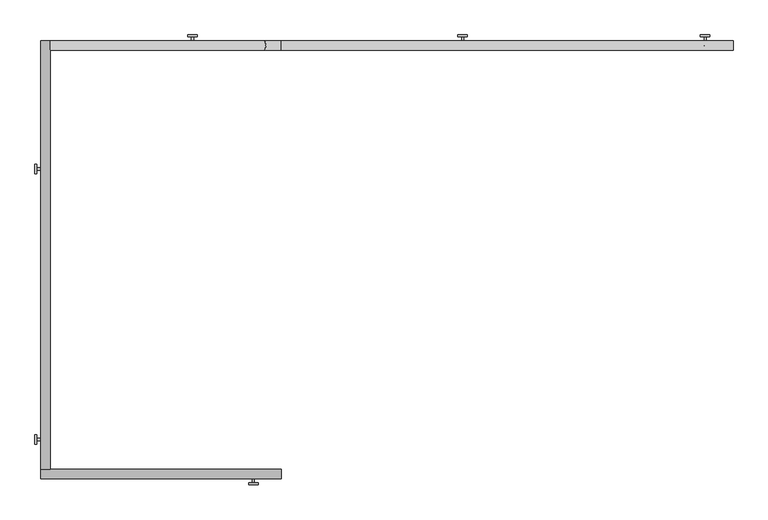
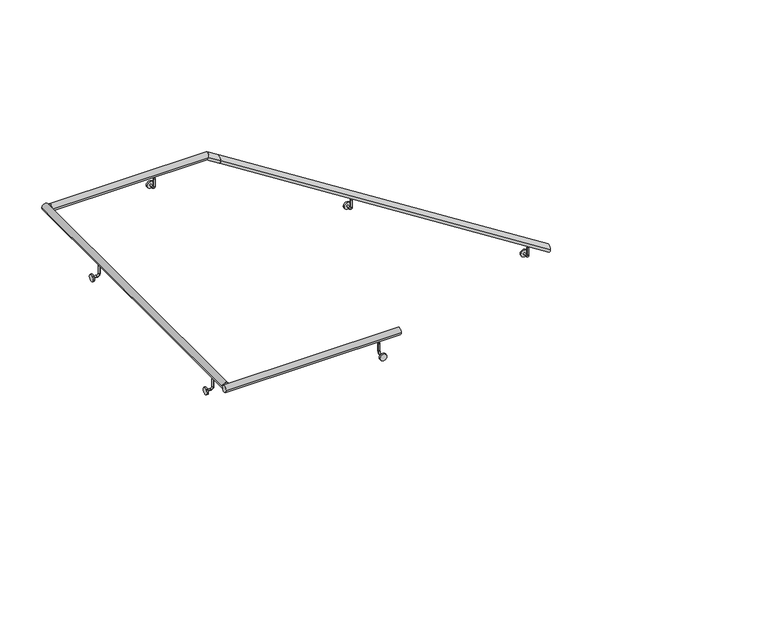
"""IFC4 building model written with IfcOpenShell, lengths in millimetres: railing geometry."""

import ifcopenshell
import ifcopenshell.guid

model = None  # the IFC model being written
_history = None  # IfcOwnerHistory: only IFC2X3 demands one
_inside = {}  # id of a spatial element -> (the spatial element, [elements in it])
_under = {}  # id of a project, library or spatial element -> (it, [spatial elements below it])
_declared = {}  # id of a project -> (the project, [libraries it declares])
_typed = {}  # id of a type object -> (the type object, [elements of that type])
_made_of = {}  # id of a material, layer set ... -> (it, [elements and type objects made of it])


def new_model(schema):
    """Start an empty IFC model of exactly this schema.

    Asked for "IFC4X3", IfcOpenShell would pick the latest addendum, in which some entities
    have other attributes; the version numbers below select the first issue.
    IFC2X3 requires an IfcOwnerHistory on every rooted entity: one is made here for all.
    """
    global model, _history
    if schema == "IFC4X3":
        model = ifcopenshell.file(schema_version=(4, 3, 0, 0))
    else:
        model = ifcopenshell.file(schema=schema)
    _inside.clear()
    _under.clear()
    _declared.clear()
    _typed.clear()
    _made_of.clear()
    _history = None
    if model.schema == "IFC2X3":
        org = make("IfcOrganization", Name="unknown")
        user = make(
            "IfcPersonAndOrganization",
            ThePerson=make("IfcPerson", FamilyName="unknown"),
            TheOrganization=org,
        )
        app = make(
            "IfcApplication",
            ApplicationDeveloper=org,
            Version="unknown",
            ApplicationFullName="unknown",
            ApplicationIdentifier="unknown",
        )
        _history = make(
            "IfcOwnerHistory",
            OwningUser=user,
            OwningApplication=app,
            ChangeAction="ADDED",
            CreationDate=0,
        )
    return model


def make(cls, **values):
    """One entity of the class cls with the attributes given. An attribute that is None is left unset."""
    return model.create_entity(
        cls, **{name: value for name, value in values.items() if value is not None}
    )


def rooted(cls, **values):
    """An entity with a GlobalId (a new one), such as an element, a storey or a relation."""
    return make(cls, GlobalId=ifcopenshell.guid.new(), OwnerHistory=_history, **values)


def si_unit(unit_type, name, prefix=None):
    """IfcSIUnit, for example si_unit("LENGTHUNIT", "METRE", prefix="MILLI")."""
    return make("IfcSIUnit", UnitType=unit_type, Prefix=prefix, Name=name)


def assignment(units):
    """IfcUnitAssignment: the units of a project."""
    return None if units is None else make("IfcUnitAssignment", Units=units)


def point(xyz):
    """IfcCartesianPoint."""
    return None if xyz is None else make("IfcCartesianPoint", Coordinates=xyz)


def direction(xyz):
    """IfcDirection."""
    return None if xyz is None else make("IfcDirection", DirectionRatios=xyz)


def frame(location, z_axis=None, x_axis=None):
    """IfcAxis2Placement3D, a coordinate frame: its origin and axes. An axis left out is left unset."""
    return make(
        "IfcAxis2Placement3D",
        Location=point(location),
        Axis=direction(z_axis),
        RefDirection=direction(x_axis),
    )


def frame_2d(location, x_axis=None):
    """IfcAxis2Placement2D, a coordinate frame in the plane: its origin and x axis."""
    return make(
        "IfcAxis2Placement2D", Location=point(location), RefDirection=direction(x_axis)
    )


def origin():
    """The frame at (0, 0, 0) with its axes left unset."""
    return frame((0.0, 0.0, 0.0))


def place(relative_to, where):
    """IfcLocalPlacement: puts the frame where relative to a parent placement (None: the world)."""
    return make(
        "IfcLocalPlacement", PlacementRelTo=relative_to, RelativePlacement=where
    )


def context(
    kind, dimensions, precision=None, world=None, true_north=None, identifier=None
):
    """IfcGeometricRepresentationContext, for example the 3D "Model" context."""
    return make(
        "IfcGeometricRepresentationContext",
        ContextIdentifier=identifier,
        ContextType=kind,
        CoordinateSpaceDimension=dimensions,
        Precision=precision,
        WorldCoordinateSystem=world,
        TrueNorth=true_north,
    )


def project(units=None, contexts=None):
    """IfcProject with its units and contexts."""
    return rooted(
        "IfcProject",
        Name="project",
        RepresentationContexts=contexts,
        UnitsInContext=assignment(units),
    )


def spatial(cls, under=None, at=None, **own):
    """A site, building, storey or space (cls), placed at a placement, below another one or the project."""
    s = rooted(cls, ObjectPlacement=at, **own)
    if under is not None:
        _under.setdefault(under.id(), (under, []))[1].append(s)
    return s


def circle_curve(where, radius):
    """IfcCircle in the frame where."""
    return make("IfcCircle", Position=where, Radius=radius)


def ellipse_curve(where, semi_axis1, semi_axis2):
    """IfcEllipse in the frame where."""
    return make(
        "IfcEllipse", Position=where, SemiAxis1=semi_axis1, SemiAxis2=semi_axis2
    )


def trimmed(basis, trim1, trim2, sense, master):
    """IfcTrimmedCurve: the piece of a basis curve between two trims."""
    return make(
        "IfcTrimmedCurve",
        BasisCurve=basis,
        Trim1=trim1,
        Trim2=trim2,
        SenseAgreement=sense,
        MasterRepresentation=master,
    )


def segment(curve, same_sense, transition):
    """IfcCompositeCurveSegment."""
    return make(
        "IfcCompositeCurveSegment",
        Transition=transition,
        SameSense=same_sense,
        ParentCurve=curve,
    )


def composite_curve(segments, self_intersect=None):
    """IfcCompositeCurve: segments joined end to end."""
    return make("IfcCompositeCurve", Segments=segments, SelfIntersect=self_intersect)


def outline(outer, holes=None, kind="AREA"):
    """IfcArbitraryClosedProfileDef: a profile drawn as a closed curve; with holes, ...WithVoids."""
    if holes is None:
        return make("IfcArbitraryClosedProfileDef", ProfileType=kind, OuterCurve=outer)
    return make(
        "IfcArbitraryProfileDefWithVoids",
        ProfileType=kind,
        OuterCurve=outer,
        InnerCurves=holes,
    )


def extrude(swept, where, along, depth):
    """IfcExtrudedAreaSolid: the profile swept, set in the frame where, extruded along a direction by depth."""
    return make(
        "IfcExtrudedAreaSolid",
        SweptArea=swept,
        Position=where,
        ExtrudedDirection=direction(along),
        Depth=depth,
    )


def shape(context_of_items, identifier, shape_type, items):
    """IfcShapeRepresentation: the items that make up one representation, for example the "Body"."""
    return make(
        "IfcShapeRepresentation",
        ContextOfItems=context_of_items,
        RepresentationIdentifier=identifier,
        RepresentationType=shape_type,
        Items=items,
    )


def source(mapping_origin, context_of_items, identifier, shape_type, items):
    """IfcRepresentationMap: a shape defined once, which mapped items show again and again."""
    return make(
        "IfcRepresentationMap",
        MappingOrigin=mapping_origin,
        MappedRepresentation=shape(context_of_items, identifier, shape_type, items),
    )


def transform(
    local_origin,
    x_axis=None,
    y_axis=None,
    z_axis=None,
    scale=None,
    scale2=None,
    scale3=None,
    uniform=True,
):
    """IfcCartesianTransformationOperator3D, or its non-uniform kind. x_axis, y_axis, z_axis: its Axis1, 2, 3."""
    if uniform:
        return make(
            "IfcCartesianTransformationOperator3D",
            Axis1=direction(x_axis),
            Axis2=direction(y_axis),
            LocalOrigin=point(local_origin),
            Scale=scale,
            Axis3=direction(z_axis),
        )
    return make(
        "IfcCartesianTransformationOperator3DnonUniform",
        Axis1=direction(x_axis),
        Axis2=direction(y_axis),
        LocalOrigin=point(local_origin),
        Scale=scale,
        Axis3=direction(z_axis),
        Scale2=scale2,
        Scale3=scale3,
    )


def mapped(mapping_source, mapping_target):
    """IfcMappedItem: shows the shape of a source again, moved by a transform."""
    return make(
        "IfcMappedItem", MappingSource=mapping_source, MappingTarget=mapping_target
    )


def made_of(thing, what):
    """Note that an element or type object is made of a material, layer set ...; save() writes the relation."""
    if what is not None:
        _made_of.setdefault(what.id(), (what, []))[1].append(thing)
    return thing


def element(
    cls,
    number,
    at=None,
    inside=None,
    cuts=None,
    type_object=None,
    material=None,
    context=None,
    identifier="Body",
    shape_type=None,
    held_by="IfcProductDefinitionShape",
    body=None,
    shapes=None,
    **own,
):
    """One element of the class cls, such as IfcWall. Its Tag is "e" and its number.

    at: its placement. inside: the storey or other place that contains it. cuts: it is an
    opening in that element (IfcRelVoidsElement). A single representation is given by context,
    identifier, shape_type and body (its items); several are given by shapes. held_by: the class
    of the entity that holds the representations. save() writes the other relations.
    """
    e = rooted(cls, Tag="e%d" % number, ObjectPlacement=at, **own)
    if body is not None:
        shapes = [shape(context, identifier, shape_type, body)]
    if shapes is not None:
        e.Representation = make(held_by, Representations=shapes)
    if inside is not None:
        _inside.setdefault(inside.id(), (inside, []))[1].append(e)
    if cuts is not None:
        rooted(
            "IfcRelVoidsElement", RelatingBuildingElement=cuts, RelatedOpeningElement=e
        )
    if type_object is not None:
        _typed.setdefault(type_object.id(), (type_object, []))[1].append(e)
    return made_of(e, material)


def aggregate(whole, parts):
    """IfcRelAggregates: a whole, such as a stair, and the parts it consists of."""
    return rooted("IfcRelAggregates", RelatingObject=whole, RelatedObjects=parts)


def save(model, path):
    """Write the relations noted so far, then the file.

    IfcRelAggregates (storeys below a building ...), IfcRelContainedInSpatialStructure (elements
    in a storey), IfcRelDefinesByType, IfcRelAssociatesMaterial and IfcRelDeclares: one each for
    every whole, place, type object, material and project.
    """
    for whole, parts in _under.values():
        aggregate(whole, parts)
    for where, things in _inside.values():
        rooted(
            "IfcRelContainedInSpatialStructure",
            RelatedElements=things,
            RelatingStructure=where,
        )
    for kind, things in _typed.values():
        rooted("IfcRelDefinesByType", RelatedObjects=things, RelatingType=kind)
    for what, things in _made_of.values():
        rooted("IfcRelAssociatesMaterial", RelatedObjects=things, RelatingMaterial=what)
    for by, libraries in _declared.values():
        rooted("IfcRelDeclares", RelatingContext=by, RelatedDefinitions=libraries)
    model.write(path)


def plane_surface(at):
    """IfcPlane: the flat surface through the origin of the frame at, square to its z axis."""
    return make("IfcPlane", Position=at)


def cylinder_surface(at, radius):
    """IfcCylindricalSurface: all points at the distance radius from the z axis of the frame at."""
    return make("IfcCylindricalSurface", Position=at, Radius=radius)


def revolved_surface(curve, axis_point, axis_direction):
    """IfcSurfaceOfRevolution: the curve turned about the line through axis_point along axis_direction."""
    return make(
        "IfcSurfaceOfRevolution",
        SweptCurve=make("IfcArbitraryOpenProfileDef", ProfileType="CURVE", Curve=curve),
        AxisPosition=make("IfcAxis1Placement", Location=point(axis_point), Axis=direction(axis_direction)),
    )


def advanced_brep(points, edges, surfaces, faces):
    """IfcAdvancedBrep: a solid bounded by faces that lie on surfaces and meet in shared edges.

    An edge is (start, end): straight between two places in points (the first is 0);
    or (start, end, curve); or (start, end, curve, False) where it runs against its curve.
    A face is (place in surfaces, loops), or (place, loops, False) where it looks against
    its surface's normal. A loop lists edges by number (the first is 1), with a minus sign
    where the edge is run from its end to its start. The first loop is the outer one.
    """
    corners = [point(p) for p in points]
    vertices = [make("IfcVertexPoint", VertexGeometry=c) for c in corners]
    made = []
    for start, end, *more in edges:
        made.append(
            make(
                "IfcEdgeCurve",
                EdgeStart=vertices[start],
                EdgeEnd=vertices[end],
                EdgeGeometry=more[0] if more else make("IfcPolyline", Points=[corners[start], corners[end]]),
                SameSense=more[1] if len(more) > 1 else True,
            )
        )
    hull = []
    for where, loops, *sense in faces:
        bounds = []
        for j, loop in enumerate(loops):
            ring = [make("IfcOrientedEdge", EdgeElement=made[abs(k) - 1], Orientation=k > 0) for k in loop]
            bounds.append(
                make(
                    "IfcFaceOuterBound" if j == 0 else "IfcFaceBound",
                    Bound=make("IfcEdgeLoop", EdgeList=ring),
                    Orientation=True,
                )
            )
        hull.append(make("IfcAdvancedFace", Bounds=bounds, FaceSurface=surfaces[where], SameSense=sense[0] if sense else True))
    return make("IfcAdvancedBrep", Outer=make("IfcClosedShell", CfsFaces=hull))


def railing_d584f0b8(model_context):
    return source(origin(), model_context, "Body", "SolidModel", [
        advanced_brep(
        [(-47747.4858495, 17739.1574868, 4652.1467196), (-47747.4858495, 17789.1574868, 4652.1467196), (-50177.4858495, 17739.1574868, 6195.0038624), (-50177.4858495, 17789.1574868, 6195.0038624)],
        [
            (0, 1, ellipse_curve(frame((-47747.4858495, 17764.1574868, 4652.1467196), z_axis=(1.0, 0.0, 0.0), x_axis=(0.0, 0.0, -1.0)), 29.613386, 25.0)),
            (1, 0, ellipse_curve(frame((-47747.4858495, 17764.1574868, 4652.1467196), z_axis=(1.0, 0.0, 0.0), x_axis=(0.0, 0.0, -1.0)), 29.613386, 25.0)),
            (2, 3, ellipse_curve(frame((-50177.4858495, 17764.1574868, 6195.0038624), z_axis=(-1.0, 0.0, 0.0), x_axis=(0.0, 0.0, -1.0)), 29.613386, 25.0)),
            (3, 2, ellipse_curve(frame((-50177.4858495, 17764.1574868, 6195.0038624), z_axis=(-1.0, 0.0, 0.0), x_axis=(0.0, 0.0, -1.0)), 29.613386, 25.0)),
            (0, 2),
            (3, 1),
        ],
        [
            plane_surface(frame((-47747.4858495, 17764.1574868, 4681.7601056), z_axis=(1.0, 0.0, 0.0), x_axis=(0.0, -1.0, 0.0))),
            plane_surface(frame((-50177.4858495, 17764.1574868, 6224.6172485), z_axis=(-1.0, 0.0, 0.0), x_axis=(0.0, -1.0, 0.0))),
            cylinder_surface(frame((-47760.8860529, 17764.1574868, 4660.6547852), z_axis=(0.8442128152478047, 0.0, -0.5360081366652713), x_axis=(0.0, 1.0, 0.0)), 25.0),
        ],
        [
            (0, [[1, 2]]),
            (1, [[3, 4]]),
            (2, [[-1, 5, -4, 6]]),
            (2, [[-2, -6, -3, -5]]),
        ],
    ),
        advanced_brep(
        [(-50177.4858495, 17739.1574868, 6195.0038624), (-50177.4858495, 17789.1574868, 6195.0038624), (-50268.4797662, 17739.1574868, 6252.7777778), (-50268.4797662, 17789.1574868, 6252.7777778), (-51419.7848926, 17739.1574868, 6252.7777778), (-51419.7848926, 17789.1574868, 6252.7777778)],
        [
            (0, 1, ellipse_curve(frame((-50177.4858495, 17764.1574868, 6195.0038624), z_axis=(1.0, 0.0, 0.0), x_axis=(0.0, 0.0, -1.0)), 29.613386, 25.0)),
            (1, 0, ellipse_curve(frame((-50177.4858495, 17764.1574868, 6195.0038624), z_axis=(1.0, 0.0, 0.0), x_axis=(0.0, 0.0, -1.0)), 29.613386, 25.0)),
            (0, 2),
            (2, 3, ellipse_curve(frame((-50268.4797662, 17764.1574868, 6252.7777778), z_axis=(0.9602637177483601, 0.0, -0.27909423565544655), x_axis=(-0.2790942356554468, 0.0, -0.9602637177483601)), 26.0345148, 25.0)),
            (3, 1),
            (3, 2, ellipse_curve(frame((-50268.4797662, 17764.1574868, 6252.7777778), z_axis=(0.9602637177483601, 0.0, -0.27909423565544655), x_axis=(-0.2790942356554468, 0.0, -0.9602637177483601)), 26.0345148, 25.0)),
            (4, 5, circle_curve(frame((-51419.7848926, 17764.1574868, 6252.7777778), z_axis=(-1.0, 0.0, 0.0), x_axis=(0.0, 1.0, 0.0)), 25.0)),
            (5, 4, circle_curve(frame((-51419.7848926, 17764.1574868, 6252.7777778), z_axis=(-1.0, 0.0, 0.0), x_axis=(0.0, 1.0, 0.0)), 25.0)),
            (2, 4),
            (5, 3),
        ],
        [
            plane_surface(frame((-50177.4858495, 17764.1574868, 6224.6172485), z_axis=(1.0, 0.0, 0.0), x_axis=(0.0, -1.0, 0.0))),
            cylinder_surface(frame((-50190.8860529, 17764.1574868, 6203.5119281), z_axis=(0.844212815247804, 0.0, -0.5360081366652723), x_axis=(0.0, 1.0, 0.0)), 25.0),
            plane_surface(frame((-51419.7848926, 17764.1574868, 6277.7777778), z_axis=(-1.0, 0.0, 0.0), x_axis=(0.0, -1.0, 0.0))),
            cylinder_surface(frame((-50261.2136831, 17764.1574868, 6252.7777778), z_axis=(1.0, 0.0, 0.0), x_axis=(0.0, 1.0, 0.0)), 25.0),
        ],
        [
            (0, [[1, 2]]),
            (1, [[-1, 3, 4, 5]]),
            (1, [[-2, -5, 6, -3]]),
            (2, [[7, 8]]),
            (3, [[-4, 9, -8, 10]]),
            (3, [[-6, -10, -7, -9]]),
        ],
    ),
        advanced_brep(
        [(-51419.7848926, 17789.1574868, 6252.7777778), (-51469.7848926, 17789.1574868, 6252.7777778), (-51419.7848926, 15484.3574868, 6252.7777778), (-51469.7848926, 15484.3574868, 6252.7777778)],
        [
            (0, 1, circle_curve(frame((-51444.7848926, 17789.1574868, 6252.7777778), z_axis=(0.0, 1.0, 0.0), x_axis=(-1.0, 0.0, 0.0)), 25.0)),
            (1, 0, circle_curve(frame((-51444.7848926, 17789.1574868, 6252.7777778), z_axis=(0.0, 1.0, 0.0), x_axis=(-1.0, 0.0, 0.0)), 25.0)),
            (2, 3, circle_curve(frame((-51444.7848926, 15484.3574868, 6252.7777778), z_axis=(0.0, -1.0, 0.0), x_axis=(-1.0, 0.0, 0.0)), 25.0)),
            (3, 2, circle_curve(frame((-51444.7848926, 15484.3574868, 6252.7777778), z_axis=(0.0, -1.0, 0.0), x_axis=(-1.0, 0.0, 0.0)), 25.0)),
            (0, 2),
            (3, 1),
        ],
        [
            plane_surface(frame((-51444.7848926, 17789.1574868, 6277.7777778), z_axis=(0.0, 1.0, 0.0), x_axis=(0.0, 0.0, -1.0))),
            plane_surface(frame((-51444.7848926, 15484.3574868, 6277.7777778), z_axis=(0.0, -1.0, 0.0), x_axis=(0.0, 0.0, -1.0))),
            cylinder_surface(frame((-51444.7848926, 17789.1574868, 6252.7777778), z_axis=(0.0, 1.0, 0.0), x_axis=(-1.0, 0.0, 0.0)), 25.0),
        ],
        [
            (0, [[1, 2]]),
            (1, [[3, 4]]),
            (2, [[-1, 5, -4, 6]]),
            (2, [[-2, -6, -3, -5]]),
        ],
    ),
        advanced_brep(
        [(-51469.7848926, 15484.3574868, 6252.7777778), (-51469.7848926, 15434.3574868, 6252.7777778), (-50177.4858495, 15484.3574868, 6252.7777778), (-50177.4858495, 15434.3574868, 6252.7777778)],
        [
            (0, 1, circle_curve(frame((-51469.7848926, 15459.3574868, 6252.7777778), z_axis=(-1.0, 0.0, 0.0), x_axis=(0.0, -1.0, 0.0)), 25.0)),
            (1, 0, circle_curve(frame((-51469.7848926, 15459.3574868, 6252.7777778), z_axis=(-1.0, 0.0, 0.0), x_axis=(0.0, -1.0, 0.0)), 25.0)),
            (2, 3, circle_curve(frame((-50177.4858495, 15459.3574868, 6252.7777778), z_axis=(1.0, 0.0, 0.0), x_axis=(0.0, -1.0, 0.0)), 25.0)),
            (3, 2, circle_curve(frame((-50177.4858495, 15459.3574868, 6252.7777778), z_axis=(1.0, 0.0, 0.0), x_axis=(0.0, -1.0, 0.0)), 25.0)),
            (0, 2),
            (3, 1),
        ],
        [
            plane_surface(frame((-51469.7848926, 15459.3574868, 6277.7777778), z_axis=(-1.0, 0.0, 0.0), x_axis=(0.0, 1.0, 0.0))),
            plane_surface(frame((-50177.4858495, 15459.3574868, 6277.7777778), z_axis=(1.0, 0.0, 0.0), x_axis=(0.0, 1.0, 0.0))),
            cylinder_surface(frame((-51469.7848926, 15459.3574868, 6252.7777778), z_axis=(-1.0, 0.0, 0.0), x_axis=(0.0, -1.0, 0.0)), 25.0),
        ],
        [
            (0, [[1, 2]]),
            (1, [[3, 4]]),
            (2, [[-1, 5, -4, 6]]),
            (2, [[-2, -6, -3, -5]]),
        ],
    ),
        advanced_brep(
        [(-51444.7848926, 15652.288061, 6208.7277778), (-51444.7848926, 15639.588061, 6208.7277778), (-51444.7848926, 15652.288061, 6151.5777778), (-51444.7848926, 15639.588061, 6151.5777778), (-51463.8348926, 15639.588061, 6132.5277778), (-51463.8348926, 15652.288061, 6132.5277778), (-51492.4098926, 15652.288061, 6132.5277778), (-51492.4098926, 15639.588061, 6132.5277778)],
        [
            (0, 1, circle_curve(frame((-51444.7848926, 15645.938061, 6208.7277778), z_axis=(0.0, 0.0, 1.0), x_axis=(0.0, -1.0, 0.0)), 6.35)),
            (1, 0, circle_curve(frame((-51444.7848926, 15645.938061, 6208.7277778), z_axis=(0.0, 0.0, 1.0), x_axis=(0.0, -1.0, 0.0)), 6.35)),
            (0, 2),
            (2, 3, circle_curve(frame((-51444.7848926, 15645.938061, 6151.5777778), z_axis=(0.0, 0.0, 1.0), x_axis=(0.0, -1.0, 0.0)), 6.35)),
            (3, 1),
            (3, 2, circle_curve(frame((-51444.7848926, 15645.938061, 6151.5777778), z_axis=(0.0, 0.0, 1.0), x_axis=(0.0, -1.0, 0.0)), 6.35)),
            (4, 3, circle_curve(frame((-51463.8348926, 15639.588061, 6151.5777778), z_axis=(0.0, -1.0, 0.0), x_axis=(1.0, 0.0, 0.0)), 19.05)),
            (2, 5, circle_curve(frame((-51463.8348926, 15652.288061, 6151.5777778), z_axis=(0.0, 1.0, 0.0), x_axis=(1.0, 0.0, 0.0)), 19.05)),
            (5, 4, circle_curve(frame((-51463.8348926, 15645.938061, 6132.5277778), z_axis=(1.0, 0.0, 0.0), x_axis=(0.0, -1.0, 0.0)), 6.35)),
            (4, 5, circle_curve(frame((-51463.8348926, 15645.938061, 6132.5277778), z_axis=(1.0, 0.0, 0.0), x_axis=(0.0, -1.0, 0.0)), 6.35)),
            (6, 7, circle_curve(frame((-51492.4098926, 15645.938061, 6132.5277778), z_axis=(-1.0, 0.0, 0.0), x_axis=(0.0, -1.0, 0.0)), 6.35)),
            (7, 6, circle_curve(frame((-51492.4098926, 15645.938061, 6132.5277778), z_axis=(-1.0, 0.0, 0.0), x_axis=(0.0, -1.0, 0.0)), 6.35)),
            (5, 6),
            (7, 4),
        ],
        [
            plane_surface(frame((-51444.7848926, 15639.588061, 6208.7277778), z_axis=(0.0, 0.0, 1.0), x_axis=(-1.0, 0.0, 0.0))),
            cylinder_surface(frame((-51444.7848926, 15645.938061, 6208.7277778), z_axis=(0.0, 0.0, 1.0), x_axis=(0.0, -1.0, 0.0)), 6.35),
            revolved_surface(trimmed(ellipse_curve(frame((-51444.7848926, 15645.938061, 6151.5777778), z_axis=(0.0, 0.0, 1.0), x_axis=(0.0, -1.0, 0.0)), 6.35, 6.35), [point((-51444.7848926, 15652.288061, 6151.5777778))], [point((-51444.7848926, 15639.588061, 6151.5777778))], True, "CARTESIAN"), (-51463.8348926, 15645.938061, 6151.5777778), (0.0, 1.0, 0.0)),
            revolved_surface(trimmed(ellipse_curve(frame((-51444.7848926, 15645.938061, 6151.5777778), z_axis=(0.0, 0.0, 1.0), x_axis=(0.0, -1.0, 0.0)), 6.35, 6.35), [point((-51444.7848926, 15639.588061, 6151.5777778))], [point((-51444.7848926, 15652.288061, 6151.5777778))], True, "CARTESIAN"), (-51463.8348926, 15645.938061, 6151.5777778), (0.0, 1.0, 0.0)),
            plane_surface(frame((-51492.4098926, 15645.938061, 6126.1777778), z_axis=(-1.0, 0.0, 0.0), x_axis=(0.0, -1.0, 0.0))),
            cylinder_surface(frame((-51463.8348926, 15645.938061, 6132.5277778), z_axis=(1.0, 0.0, 0.0), x_axis=(0.0, -1.0, 0.0)), 6.35),
        ],
        [
            (0, [[1, 2]]),
            (1, [[-1, 3, 4, 5]]),
            (1, [[-2, -5, 6, -3]]),
            (2, [[7, -4, 8, 9]]),
            (3, [[-8, -6, -7, 10]]),
            (4, [[11, 12]]),
            (5, [[-9, 13, -12, 14]]),
            (5, [[-10, -14, -11, -13]]),
        ],
    ),
        extrude(outline(composite_curve([segment(trimmed(circle_curve(frame_2d((15645.938061, 6132.5277778)), 25.4), [point((15620.538061, 6132.5277778))], [point((15671.338061, 6132.5277778))], False, "CARTESIAN"), True, "CONTINUOUS"), segment(trimmed(circle_curve(frame_2d((15645.938061, 6132.5277778)), 25.4), [point((15671.338061, 6132.5277778))], [point((15620.538061, 6132.5277778))], False, "CARTESIAN"), True, "CONTINUOUS")], self_intersect=False)), frame((-51501.9348926, 0.0, 0.0), z_axis=(1.0, 0.0, 0.0), x_axis=(0.0, 1.0, 0.0)), (0.0, 0.0, 1.0), 9.525),
        advanced_brep(
        [(-51444.7848926, 17106.1676782, 6208.7277778), (-51444.7848926, 17093.4676782, 6208.7277778), (-51444.7848926, 17106.1676782, 6151.5777778), (-51444.7848926, 17093.4676782, 6151.5777778), (-51463.8348926, 17093.4676782, 6132.5277778), (-51463.8348926, 17106.1676782, 6132.5277778), (-51492.4098926, 17106.1676782, 6132.5277778), (-51492.4098926, 17093.4676782, 6132.5277778)],
        [
            (0, 1, circle_curve(frame((-51444.7848926, 17099.8176782, 6208.7277778), z_axis=(0.0, 0.0, 1.0), x_axis=(0.0, -1.0, 0.0)), 6.35)),
            (1, 0, circle_curve(frame((-51444.7848926, 17099.8176782, 6208.7277778), z_axis=(0.0, 0.0, 1.0), x_axis=(0.0, -1.0, 0.0)), 6.35)),
            (0, 2),
            (2, 3, circle_curve(frame((-51444.7848926, 17099.8176782, 6151.5777778), z_axis=(0.0, 0.0, 1.0), x_axis=(0.0, -1.0, 0.0)), 6.35)),
            (3, 1),
            (3, 2, circle_curve(frame((-51444.7848926, 17099.8176782, 6151.5777778), z_axis=(0.0, 0.0, 1.0), x_axis=(0.0, -1.0, 0.0)), 6.35)),
            (4, 3, circle_curve(frame((-51463.8348926, 17093.4676782, 6151.5777778), z_axis=(0.0, -1.0, 0.0), x_axis=(1.0, 0.0, 0.0)), 19.05)),
            (2, 5, circle_curve(frame((-51463.8348926, 17106.1676782, 6151.5777778), z_axis=(0.0, 1.0, 0.0), x_axis=(1.0, 0.0, 0.0)), 19.05)),
            (5, 4, circle_curve(frame((-51463.8348926, 17099.8176782, 6132.5277778), z_axis=(1.0, 0.0, 0.0), x_axis=(0.0, -1.0, 0.0)), 6.35)),
            (4, 5, circle_curve(frame((-51463.8348926, 17099.8176782, 6132.5277778), z_axis=(1.0, 0.0, 0.0), x_axis=(0.0, -1.0, 0.0)), 6.35)),
            (6, 7, circle_curve(frame((-51492.4098926, 17099.8176782, 6132.5277778), z_axis=(-1.0, 0.0, 0.0), x_axis=(0.0, -1.0, 0.0)), 6.35)),
            (7, 6, circle_curve(frame((-51492.4098926, 17099.8176782, 6132.5277778), z_axis=(-1.0, 0.0, 0.0), x_axis=(0.0, -1.0, 0.0)), 6.35)),
            (5, 6),
            (7, 4),
        ],
        [
            plane_surface(frame((-51444.7848926, 17093.4676782, 6208.7277778), z_axis=(0.0, 0.0, 1.0), x_axis=(-1.0, 0.0, 0.0))),
            cylinder_surface(frame((-51444.7848926, 17099.8176782, 6208.7277778), z_axis=(0.0, 0.0, 1.0), x_axis=(0.0, -1.0, 0.0)), 6.35),
            revolved_surface(trimmed(ellipse_curve(frame((-51444.7848926, 17099.8176782, 6151.5777778), z_axis=(0.0, 0.0, 1.0), x_axis=(0.0, -1.0, 0.0)), 6.35, 6.35), [point((-51444.7848926, 17106.1676782, 6151.5777778))], [point((-51444.7848926, 17093.4676782, 6151.5777778))], True, "CARTESIAN"), (-51463.8348926, 17099.8176782, 6151.5777778), (0.0, 1.0, 0.0)),
            revolved_surface(trimmed(ellipse_curve(frame((-51444.7848926, 17099.8176782, 6151.5777778), z_axis=(0.0, 0.0, 1.0), x_axis=(0.0, -1.0, 0.0)), 6.35, 6.35), [point((-51444.7848926, 17093.4676782, 6151.5777778))], [point((-51444.7848926, 17106.1676782, 6151.5777778))], True, "CARTESIAN"), (-51463.8348926, 17099.8176782, 6151.5777778), (0.0, 1.0, 0.0)),
            plane_surface(frame((-51492.4098926, 17099.8176782, 6126.1777778), z_axis=(-1.0, 0.0, 0.0), x_axis=(0.0, -1.0, 0.0))),
            cylinder_surface(frame((-51463.8348926, 17099.8176782, 6132.5277778), z_axis=(1.0, 0.0, 0.0), x_axis=(0.0, -1.0, 0.0)), 6.35),
        ],
        [
            (0, [[1, 2]]),
            (1, [[-1, 3, 4, 5]]),
            (1, [[-2, -5, 6, -3]]),
            (2, [[7, -4, 8, 9]]),
            (3, [[-8, -6, -7, 10]]),
            (4, [[11, 12]]),
            (5, [[-9, 13, -12, 14]]),
            (5, [[-10, -14, -11, -13]]),
        ],
    ),
        extrude(outline(composite_curve([segment(trimmed(circle_curve(frame_2d((17099.8176782, 6132.5277778)), 25.4), [point((17074.4176782, 6132.5277778))], [point((17125.2176782, 6132.5277778))], False, "CARTESIAN"), True, "CONTINUOUS"), segment(trimmed(circle_curve(frame_2d((17099.8176782, 6132.5277778)), 25.4), [point((17125.2176782, 6132.5277778))], [point((17074.4176782, 6132.5277778))], False, "CARTESIAN"), True, "CONTINUOUS")], self_intersect=False)), frame((-51501.9348926, 0.0, 0.0), z_axis=(1.0, 0.0, 0.0), x_axis=(0.0, 1.0, 0.0)), (0.0, 0.0, 1.0), 9.525),
        advanced_brep(
        [(-50648.895084, 17764.1574868, 6208.7277778), (-50661.595084, 17764.1574868, 6208.7277778), (-50648.895084, 17764.1574868, 6151.5777778), (-50661.595084, 17764.1574868, 6151.5777778), (-50661.595084, 17783.2074868, 6132.5277778), (-50648.895084, 17783.2074868, 6132.5277778), (-50648.895084, 17811.7824868, 6132.5277778), (-50661.595084, 17811.7824868, 6132.5277778)],
        [
            (0, 1, circle_curve(frame((-50655.245084, 17764.1574868, 6208.7277778), z_axis=(0.0, 0.0, 1.0), x_axis=(-1.0, 0.0, 0.0)), 6.35)),
            (1, 0, circle_curve(frame((-50655.245084, 17764.1574868, 6208.7277778), z_axis=(0.0, 0.0, 1.0), x_axis=(-1.0, 0.0, 0.0)), 6.35)),
            (0, 2),
            (2, 3, circle_curve(frame((-50655.245084, 17764.1574868, 6151.5777778), z_axis=(0.0, 0.0, 1.0), x_axis=(-1.0, 0.0, 0.0)), 6.35)),
            (3, 1),
            (3, 2, circle_curve(frame((-50655.245084, 17764.1574868, 6151.5777778), z_axis=(0.0, 0.0, 1.0), x_axis=(-1.0, 0.0, 0.0)), 6.35)),
            (4, 3, circle_curve(frame((-50661.595084, 17783.2074868, 6151.5777778), z_axis=(-1.0, 0.0, 0.0), x_axis=(0.0, -1.0, 0.0)), 19.05)),
            (2, 5, circle_curve(frame((-50648.895084, 17783.2074868, 6151.5777778), z_axis=(1.0, 0.0, 0.0), x_axis=(0.0, -1.0, 0.0)), 19.05)),
            (5, 4, circle_curve(frame((-50655.245084, 17783.2074868, 6132.5277778), z_axis=(0.0, -1.0, 0.0), x_axis=(-1.0, 0.0, 0.0)), 6.35)),
            (4, 5, circle_curve(frame((-50655.245084, 17783.2074868, 6132.5277778), z_axis=(0.0, -1.0, 0.0), x_axis=(-1.0, 0.0, 0.0)), 6.35)),
            (6, 7, circle_curve(frame((-50655.245084, 17811.7824868, 6132.5277778), z_axis=(0.0, 1.0, 0.0), x_axis=(-1.0, 0.0, 0.0)), 6.35)),
            (7, 6, circle_curve(frame((-50655.245084, 17811.7824868, 6132.5277778), z_axis=(0.0, 1.0, 0.0), x_axis=(-1.0, 0.0, 0.0)), 6.35)),
            (5, 6),
            (7, 4),
        ],
        [
            plane_surface(frame((-50661.595084, 17764.1574868, 6208.7277778), z_axis=(0.0, 0.0, 1.0), x_axis=(0.0, 1.0, 0.0))),
            cylinder_surface(frame((-50655.245084, 17764.1574868, 6208.7277778), z_axis=(0.0, 0.0, 1.0), x_axis=(-1.0, 0.0, 0.0)), 6.35),
            revolved_surface(trimmed(ellipse_curve(frame((-50655.245084, 17764.1574868, 6151.5777778), z_axis=(0.0, 0.0, 1.0), x_axis=(-1.0, 0.0, 0.0)), 6.35, 6.35), [point((-50648.895084, 17764.1574868, 6151.5777778))], [point((-50661.595084, 17764.1574868, 6151.5777778))], True, "CARTESIAN"), (-50655.245084, 17783.2074868, 6151.5777778), (1.0, 0.0, 0.0)),
            revolved_surface(trimmed(ellipse_curve(frame((-50655.245084, 17764.1574868, 6151.5777778), z_axis=(0.0, 0.0, 1.0), x_axis=(-1.0, 0.0, 0.0)), 6.35, 6.35), [point((-50661.595084, 17764.1574868, 6151.5777778))], [point((-50648.895084, 17764.1574868, 6151.5777778))], True, "CARTESIAN"), (-50655.245084, 17783.2074868, 6151.5777778), (1.0, 0.0, 0.0)),
            plane_surface(frame((-50655.245084, 17811.7824868, 6126.1777778), z_axis=(0.0, 1.0, 0.0), x_axis=(-1.0, 0.0, 0.0))),
            cylinder_surface(frame((-50655.245084, 17783.2074868, 6132.5277778), z_axis=(0.0, -1.0, 0.0), x_axis=(-1.0, 0.0, 0.0)), 6.35),
        ],
        [
            (0, [[1, 2]]),
            (1, [[-1, 3, 4, 5]]),
            (1, [[-2, -5, 6, -3]]),
            (2, [[7, -4, 8, 9]]),
            (3, [[-8, -6, -7, 10]]),
            (4, [[11, 12]]),
            (5, [[-9, 13, -12, 14]]),
            (5, [[-10, -14, -11, -13]]),
        ],
    ),
        extrude(outline(composite_curve([segment(trimmed(circle_curve(frame_2d((6132.5277778, -50655.245084)), 25.4), [point((6132.5277778, -50680.645084))], [point((6132.5277778, -50629.845084))], False, "CARTESIAN"), True, "CONTINUOUS"), segment(trimmed(circle_curve(frame_2d((6132.5277778, -50655.245084)), 25.4), [point((6132.5277778, -50629.845084))], [point((6132.5277778, -50680.645084))], False, "CARTESIAN"), True, "CONTINUOUS")], self_intersect=False)), frame((0.0, 17811.7824868, 0.0), z_axis=(0.0, 1.0, 0.0), x_axis=(0.0, 0.0, 1.0)), (0.0, 0.0, 1.0), 9.525),
        advanced_brep(
        [(-49195.0154667, 17764.1574868, 5535.8082753), (-49207.7154667, 17764.1574868, 5535.8082753), (-49195.0154667, 17764.1574868, 5478.6582753), (-49207.7154667, 17764.1574868, 5478.6582753), (-49207.7154667, 17783.2074868, 5459.6082753), (-49195.0154667, 17783.2074868, 5459.6082753), (-49195.0154667, 17811.7824868, 5459.6082753), (-49207.7154667, 17811.7824868, 5459.6082753)],
        [
            (0, 1, circle_curve(frame((-49201.3654667, 17764.1574868, 5535.8082753), z_axis=(0.0, 0.0, 1.0), x_axis=(-1.0, 0.0, 0.0)), 6.35)),
            (1, 0, circle_curve(frame((-49201.3654667, 17764.1574868, 5535.8082753), z_axis=(0.0, 0.0, 1.0), x_axis=(-1.0, 0.0, 0.0)), 6.35)),
            (0, 2),
            (2, 3, circle_curve(frame((-49201.3654667, 17764.1574868, 5478.6582753), z_axis=(0.0, 0.0, 1.0), x_axis=(-1.0, 0.0, 0.0)), 6.35)),
            (3, 1),
            (3, 2, circle_curve(frame((-49201.3654667, 17764.1574868, 5478.6582753), z_axis=(0.0, 0.0, 1.0), x_axis=(-1.0, 0.0, 0.0)), 6.35)),
            (4, 3, circle_curve(frame((-49207.7154667, 17783.2074868, 5478.6582753), z_axis=(-1.0, 0.0, 0.0), x_axis=(0.0, -1.0, 0.0)), 19.05)),
            (2, 5, circle_curve(frame((-49195.0154667, 17783.2074868, 5478.6582753), z_axis=(1.0, 0.0, 0.0), x_axis=(0.0, -1.0, 0.0)), 19.05)),
            (5, 4, circle_curve(frame((-49201.3654667, 17783.2074868, 5459.6082753), z_axis=(0.0, -1.0, 0.0), x_axis=(-1.0, 0.0, 0.0)), 6.35)),
            (4, 5, circle_curve(frame((-49201.3654667, 17783.2074868, 5459.6082753), z_axis=(0.0, -1.0, 0.0), x_axis=(-1.0, 0.0, 0.0)), 6.35)),
            (6, 7, circle_curve(frame((-49201.3654667, 17811.7824868, 5459.6082753), z_axis=(0.0, 1.0, 0.0), x_axis=(-1.0, 0.0, 0.0)), 6.35)),
            (7, 6, circle_curve(frame((-49201.3654667, 17811.7824868, 5459.6082753), z_axis=(0.0, 1.0, 0.0), x_axis=(-1.0, 0.0, 0.0)), 6.35)),
            (5, 6),
            (7, 4),
        ],
        [
            plane_surface(frame((-49207.7154667, 17764.1574868, 5535.8082753), z_axis=(0.0, 0.0, 1.0), x_axis=(0.0, 1.0, 0.0))),
            cylinder_surface(frame((-49201.3654667, 17764.1574868, 5535.8082753), z_axis=(0.0, 0.0, 1.0), x_axis=(-1.0, 0.0, 0.0)), 6.35),
            revolved_surface(trimmed(ellipse_curve(frame((-49201.3654667, 17764.1574868, 5478.6582753), z_axis=(0.0, 0.0, 1.0), x_axis=(-1.0, 0.0, 0.0)), 6.35, 6.35), [point((-49195.0154667, 17764.1574868, 5478.6582753))], [point((-49207.7154667, 17764.1574868, 5478.6582753))], True, "CARTESIAN"), (-49201.3654667, 17783.2074868, 5478.6582753), (1.0, 0.0, 0.0)),
            revolved_surface(trimmed(ellipse_curve(frame((-49201.3654667, 17764.1574868, 5478.6582753), z_axis=(0.0, 0.0, 1.0), x_axis=(-1.0, 0.0, 0.0)), 6.35, 6.35), [point((-49207.7154667, 17764.1574868, 5478.6582753))], [point((-49195.0154667, 17764.1574868, 5478.6582753))], True, "CARTESIAN"), (-49201.3654667, 17783.2074868, 5478.6582753), (1.0, 0.0, 0.0)),
            plane_surface(frame((-49201.3654667, 17811.7824868, 5453.2582753), z_axis=(0.0, 1.0, 0.0), x_axis=(-1.0, 0.0, 0.0))),
            cylinder_surface(frame((-49201.3654667, 17783.2074868, 5459.6082753), z_axis=(0.0, -1.0, 0.0), x_axis=(-1.0, 0.0, 0.0)), 6.35),
        ],
        [
            (0, [[1, 2]]),
            (1, [[-1, 3, 4, 5]]),
            (1, [[-2, -5, 6, -3]]),
            (2, [[7, -4, 8, 9]]),
            (3, [[-8, -6, -7, 10]]),
            (4, [[11, 12]]),
            (5, [[-9, 13, -12, 14]]),
            (5, [[-10, -14, -11, -13]]),
        ],
    ),
        extrude(outline(composite_curve([segment(trimmed(circle_curve(frame_2d((5459.6082753, -49201.3654667)), 25.4), [point((5459.6082753, -49226.7654667))], [point((5459.6082753, -49175.9654667))], False, "CARTESIAN"), True, "CONTINUOUS"), segment(trimmed(circle_curve(frame_2d((5459.6082753, -49201.3654667)), 25.4), [point((5459.6082753, -49175.9654667))], [point((5459.6082753, -49226.7654667))], False, "CARTESIAN"), True, "CONTINUOUS")], self_intersect=False)), frame((0.0, 17811.7824868, 0.0), z_axis=(0.0, 1.0, 0.0), x_axis=(0.0, 0.0, 1.0)), (0.0, 0.0, 1.0), 9.525),
        advanced_brep(
        [(-50333.8358495, 15459.3574868, 6208.7277778), (-50321.1358495, 15459.3574868, 6208.7277778), (-50333.8358495, 15459.3574868, 6151.5777778), (-50321.1358495, 15459.3574868, 6151.5777778), (-50321.1358495, 15440.3074868, 6132.5277778), (-50333.8358495, 15440.3074868, 6132.5277778), (-50333.8358495, 15411.7324868, 6132.5277778), (-50321.1358495, 15411.7324868, 6132.5277778)],
        [
            (0, 1, circle_curve(frame((-50327.4858495, 15459.3574868, 6208.7277778), z_axis=(0.0, 0.0, 1.0), x_axis=(1.0, 0.0, 0.0)), 6.35)),
            (1, 0, circle_curve(frame((-50327.4858495, 15459.3574868, 6208.7277778), z_axis=(0.0, 0.0, 1.0), x_axis=(1.0, 0.0, 0.0)), 6.35)),
            (0, 2),
            (2, 3, circle_curve(frame((-50327.4858495, 15459.3574868, 6151.5777778), z_axis=(0.0, 0.0, 1.0), x_axis=(1.0, 0.0, 0.0)), 6.35)),
            (3, 1),
            (3, 2, circle_curve(frame((-50327.4858495, 15459.3574868, 6151.5777778), z_axis=(0.0, 0.0, 1.0), x_axis=(1.0, 0.0, 0.0)), 6.35)),
            (4, 3, circle_curve(frame((-50321.1358495, 15440.3074868, 6151.5777778), z_axis=(1.0, 0.0, 0.0), x_axis=(0.0, 1.0, 0.0)), 19.05)),
            (2, 5, circle_curve(frame((-50333.8358495, 15440.3074868, 6151.5777778), z_axis=(-1.0, 0.0, 0.0), x_axis=(0.0, 1.0, 0.0)), 19.05)),
            (5, 4, circle_curve(frame((-50327.4858495, 15440.3074868, 6132.5277778), z_axis=(0.0, 1.0, 0.0), x_axis=(1.0, 0.0, 0.0)), 6.35)),
            (4, 5, circle_curve(frame((-50327.4858495, 15440.3074868, 6132.5277778), z_axis=(0.0, 1.0, 0.0), x_axis=(1.0, 0.0, 0.0)), 6.35)),
            (6, 7, circle_curve(frame((-50327.4858495, 15411.7324868, 6132.5277778), z_axis=(0.0, -1.0, 0.0), x_axis=(1.0, 0.0, 0.0)), 6.35)),
            (7, 6, circle_curve(frame((-50327.4858495, 15411.7324868, 6132.5277778), z_axis=(0.0, -1.0, 0.0), x_axis=(1.0, 0.0, 0.0)), 6.35)),
            (5, 6),
            (7, 4),
        ],
        [
            plane_surface(frame((-50321.1358495, 15459.3574868, 6208.7277778), z_axis=(0.0, 0.0, 1.0), x_axis=(0.0, -1.0, 0.0))),
            cylinder_surface(frame((-50327.4858495, 15459.3574868, 6208.7277778), z_axis=(0.0, 0.0, 1.0), x_axis=(1.0, 0.0, 0.0)), 6.35),
            revolved_surface(trimmed(ellipse_curve(frame((-50327.4858495, 15459.3574868, 6151.5777778), z_axis=(0.0, 0.0, 1.0), x_axis=(1.0, 0.0, 0.0)), 6.35, 6.35), [point((-50333.8358495, 15459.3574868, 6151.5777778))], [point((-50321.1358495, 15459.3574868, 6151.5777778))], True, "CARTESIAN"), (-50327.4858495, 15440.3074868, 6151.5777778), (-1.0, 0.0, 0.0)),
            revolved_surface(trimmed(ellipse_curve(frame((-50327.4858495, 15459.3574868, 6151.5777778), z_axis=(0.0, 0.0, 1.0), x_axis=(1.0, 0.0, 0.0)), 6.35, 6.35), [point((-50321.1358495, 15459.3574868, 6151.5777778))], [point((-50333.8358495, 15459.3574868, 6151.5777778))], True, "CARTESIAN"), (-50327.4858495, 15440.3074868, 6151.5777778), (-1.0, 0.0, 0.0)),
            plane_surface(frame((-50327.4858495, 15411.7324868, 6126.1777778), z_axis=(0.0, -1.0, 0.0), x_axis=(1.0, 0.0, 0.0))),
            cylinder_surface(frame((-50327.4858495, 15440.3074868, 6132.5277778), z_axis=(0.0, 1.0, 0.0), x_axis=(1.0, 0.0, 0.0)), 6.35),
        ],
        [
            (0, [[1, 2]]),
            (1, [[-1, 3, 4, 5]]),
            (1, [[-2, -5, 6, -3]]),
            (2, [[7, -4, 8, 9]]),
            (3, [[-8, -6, -7, 10]]),
            (4, [[11, 12]]),
            (5, [[-9, 13, -12, 14]]),
            (5, [[-10, -14, -11, -13]]),
        ],
    ),
        extrude(outline(composite_curve([segment(trimmed(circle_curve(frame_2d((6132.5277778, -50327.4858495)), 25.4), [point((6132.5277778, -50302.0858495))], [point((6132.5277778, -50352.8858495))], False, "CARTESIAN"), True, "CONTINUOUS"), segment(trimmed(circle_curve(frame_2d((6132.5277778, -50327.4858495)), 25.4), [point((6132.5277778, -50352.8858495))], [point((6132.5277778, -50302.0858495))], False, "CARTESIAN"), True, "CONTINUOUS")], self_intersect=False)), frame((0.0, 15402.2074868, 0.0), z_axis=(0.0, 1.0, 0.0), x_axis=(0.0, 0.0, 1.0)), (0.0, 0.0, 1.0), 9.525),
        advanced_brep(
        [(-47891.1358495, 17764.1574868, 4707.9482009), (-47903.8358495, 17764.1574868, 4707.9482009), (-47891.1358495, 17764.1574868, 4650.7982009), (-47903.8358495, 17764.1574868, 4650.7982009), (-47903.8358495, 17783.2074868, 4631.7482009), (-47891.1358495, 17783.2074868, 4631.7482009), (-47891.1358495, 17811.7824868, 4631.7482009), (-47903.8358495, 17811.7824868, 4631.7482009)],
        [
            (0, 1, circle_curve(frame((-47897.4858495, 17764.1574868, 4707.9482009), z_axis=(0.0, 0.0, 1.0), x_axis=(-1.0, 0.0, 0.0)), 6.35)),
            (1, 0, circle_curve(frame((-47897.4858495, 17764.1574868, 4707.9482009), z_axis=(0.0, 0.0, 1.0), x_axis=(-1.0, 0.0, 0.0)), 6.35)),
            (0, 2),
            (2, 3, circle_curve(frame((-47897.4858495, 17764.1574868, 4650.7982009), z_axis=(0.0, 0.0, 1.0), x_axis=(-1.0, 0.0, 0.0)), 6.35)),
            (3, 1),
            (3, 2, circle_curve(frame((-47897.4858495, 17764.1574868, 4650.7982009), z_axis=(0.0, 0.0, 1.0), x_axis=(-1.0, 0.0, 0.0)), 6.35)),
            (4, 3, circle_curve(frame((-47903.8358495, 17783.2074868, 4650.7982009), z_axis=(-1.0, 0.0, 0.0), x_axis=(0.0, -1.0, 0.0)), 19.05)),
            (2, 5, circle_curve(frame((-47891.1358495, 17783.2074868, 4650.7982009), z_axis=(1.0, 0.0, 0.0), x_axis=(0.0, -1.0, 0.0)), 19.05)),
            (5, 4, circle_curve(frame((-47897.4858495, 17783.2074868, 4631.7482009), z_axis=(0.0, -1.0, 0.0), x_axis=(-1.0, 0.0, 0.0)), 6.35)),
            (4, 5, circle_curve(frame((-47897.4858495, 17783.2074868, 4631.7482009), z_axis=(0.0, -1.0, 0.0), x_axis=(-1.0, 0.0, 0.0)), 6.35)),
            (6, 7, circle_curve(frame((-47897.4858495, 17811.7824868, 4631.7482009), z_axis=(0.0, 1.0, 0.0), x_axis=(-1.0, 0.0, 0.0)), 6.35)),
            (7, 6, circle_curve(frame((-47897.4858495, 17811.7824868, 4631.7482009), z_axis=(0.0, 1.0, 0.0), x_axis=(-1.0, 0.0, 0.0)), 6.35)),
            (5, 6),
            (7, 4),
        ],
        [
            plane_surface(frame((-47903.8358495, 17764.1574868, 4707.9482009), z_axis=(0.0, 0.0, 1.0), x_axis=(0.0, 1.0, 0.0))),
            cylinder_surface(frame((-47897.4858495, 17764.1574868, 4707.9482009), z_axis=(0.0, 0.0, 1.0), x_axis=(-1.0, 0.0, 0.0)), 6.35),
            revolved_surface(trimmed(ellipse_curve(frame((-47897.4858495, 17764.1574868, 4650.7982009), z_axis=(0.0, 0.0, 1.0), x_axis=(-1.0, 0.0, 0.0)), 6.35, 6.35), [point((-47891.1358495, 17764.1574868, 4650.7982009))], [point((-47903.8358495, 17764.1574868, 4650.7982009))], True, "CARTESIAN"), (-47897.4858495, 17783.2074868, 4650.7982009), (1.0, 0.0, 0.0)),
            revolved_surface(trimmed(ellipse_curve(frame((-47897.4858495, 17764.1574868, 4650.7982009), z_axis=(0.0, 0.0, 1.0), x_axis=(-1.0, 0.0, 0.0)), 6.35, 6.35), [point((-47903.8358495, 17764.1574868, 4650.7982009))], [point((-47891.1358495, 17764.1574868, 4650.7982009))], True, "CARTESIAN"), (-47897.4858495, 17783.2074868, 4650.7982009), (1.0, 0.0, 0.0)),
            plane_surface(frame((-47897.4858495, 17811.7824868, 4625.3982009), z_axis=(0.0, 1.0, 0.0), x_axis=(-1.0, 0.0, 0.0))),
            cylinder_surface(frame((-47897.4858495, 17783.2074868, 4631.7482009), z_axis=(0.0, -1.0, 0.0), x_axis=(-1.0, 0.0, 0.0)), 6.35),
        ],
        [
            (0, [[1, 2]]),
            (1, [[-1, 3, 4, 5]]),
            (1, [[-2, -5, 6, -3]]),
            (2, [[7, -4, 8, 9]]),
            (3, [[-8, -6, -7, 10]]),
            (4, [[11, 12]]),
            (5, [[-9, 13, -12, 14]]),
            (5, [[-10, -14, -11, -13]]),
        ],
    ),
        extrude(outline(composite_curve([segment(trimmed(circle_curve(frame_2d((4631.7482009, -47897.4858495)), 25.4), [point((4631.7482009, -47922.8858495))], [point((4631.7482009, -47872.0858495))], False, "CARTESIAN"), True, "CONTINUOUS"), segment(trimmed(circle_curve(frame_2d((4631.7482009, -47897.4858495)), 25.4), [point((4631.7482009, -47872.0858495))], [point((4631.7482009, -47922.8858495))], False, "CARTESIAN"), True, "CONTINUOUS")], self_intersect=False)), frame((0.0, 17811.7824868, 0.0), z_axis=(0.0, 1.0, 0.0), x_axis=(0.0, 0.0, 1.0)), (0.0, 0.0, 1.0), 9.525),
    ])


if __name__ == "__main__":
    model = new_model("IFC4")
    model_context = context("Model", 3, world=origin())
    ifc_project = project(units=[si_unit("LENGTHUNIT", "METRE", prefix="MILLI")], contexts=[model_context])
    site = spatial("IfcSite", under=ifc_project)
    building = spatial("IfcBuilding", under=site)
    placement = place(None, origin())
    railing_shape = railing_d584f0b8(model_context)
    element("IfcRailing", 1, at=placement, inside=building, context=model_context, shape_type="MappedRepresentation", body=[
        mapped(railing_shape, transform((0.0, 0.0, 0.0), x_axis=(1.0, 0.0, 0.0), y_axis=(0.0, 1.0, 0.0), z_axis=(0.0, 0.0, 1.0))),
    ])
    save(model, "model.ifc")

# Revit data of these elements
# Project information
#   Projekt-Nummer = "Hier die Projektnummer eintragen!"
#   IfcSite GUID = "3DdyCULLv3kQRx$MQ8PThJ"
#   IfcBuilding GUID = "3DdyCULLv3kQRx$MQ8PThG"
#   IfcProject GUID = "3DdyCULLv3kQRx$MQ8PThH"
#   Classification.Facility.Number = "Co_20_15_58"
#   Classification.Facility.Description = "Office complexes"
#   Project Status = "Projektstatus"
#   Project Address = "Geben Sie die Adresse hier ein"
